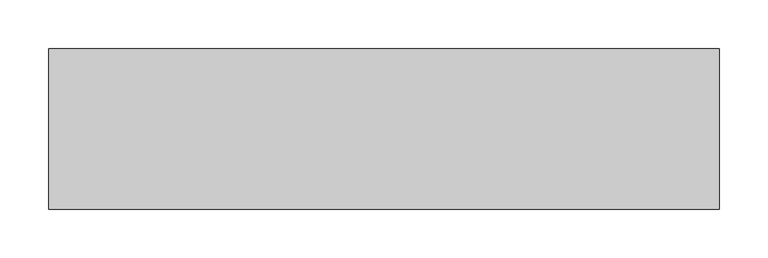
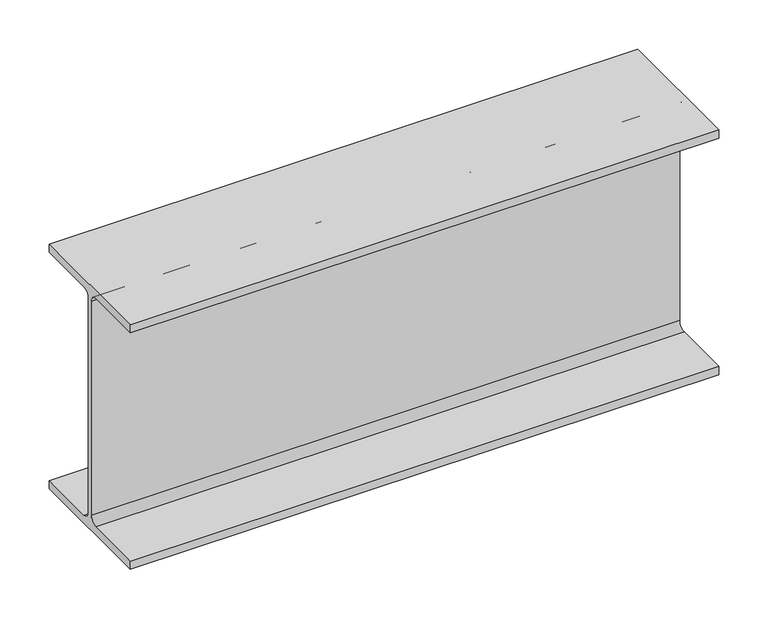
"""IFC4 building model written with IfcOpenShell, lengths in millimetres: beam geometry, Old_Steel Beam_H-KSD3502 : H_SB_ASB_H-300×150x6.5x9."""

import ifcopenshell
import ifcopenshell.guid

model = None  # the IFC model being written
_history = None  # IfcOwnerHistory: only IFC2X3 demands one
_inside = {}  # id of a spatial element -> (the spatial element, [elements in it])
_under = {}  # id of a project, library or spatial element -> (it, [spatial elements below it])
_declared = {}  # id of a project -> (the project, [libraries it declares])
_typed = {}  # id of a type object -> (the type object, [elements of that type])
_made_of = {}  # id of a material, layer set ... -> (it, [elements and type objects made of it])


def new_model(schema):
    """Start an empty IFC model of exactly this schema.

    Asked for "IFC4X3", IfcOpenShell would pick the latest addendum, in which some entities
    have other attributes; the version numbers below select the first issue.
    IFC2X3 requires an IfcOwnerHistory on every rooted entity: one is made here for all.
    """
    global model, _history
    if schema == "IFC4X3":
        model = ifcopenshell.file(schema_version=(4, 3, 0, 0))
    else:
        model = ifcopenshell.file(schema=schema)
    _inside.clear()
    _under.clear()
    _declared.clear()
    _typed.clear()
    _made_of.clear()
    _history = None
    if model.schema == "IFC2X3":
        org = make("IfcOrganization", Name="unknown")
        user = make(
            "IfcPersonAndOrganization",
            ThePerson=make("IfcPerson", FamilyName="unknown"),
            TheOrganization=org,
        )
        app = make(
            "IfcApplication",
            ApplicationDeveloper=org,
            Version="unknown",
            ApplicationFullName="unknown",
            ApplicationIdentifier="unknown",
        )
        _history = make(
            "IfcOwnerHistory",
            OwningUser=user,
            OwningApplication=app,
            ChangeAction="ADDED",
            CreationDate=0,
        )
    return model


def make(cls, **values):
    """One entity of the class cls with the attributes given. An attribute that is None is left unset."""
    return model.create_entity(
        cls, **{name: value for name, value in values.items() if value is not None}
    )


def rooted(cls, **values):
    """An entity with a GlobalId (a new one), such as an element, a storey or a relation."""
    return make(cls, GlobalId=ifcopenshell.guid.new(), OwnerHistory=_history, **values)


def si_unit(unit_type, name, prefix=None):
    """IfcSIUnit, for example si_unit("LENGTHUNIT", "METRE", prefix="MILLI")."""
    return make("IfcSIUnit", UnitType=unit_type, Prefix=prefix, Name=name)


def assignment(units):
    """IfcUnitAssignment: the units of a project."""
    return None if units is None else make("IfcUnitAssignment", Units=units)


def point(xyz):
    """IfcCartesianPoint."""
    return None if xyz is None else make("IfcCartesianPoint", Coordinates=xyz)


def direction(xyz):
    """IfcDirection."""
    return None if xyz is None else make("IfcDirection", DirectionRatios=xyz)


def frame(location, z_axis=None, x_axis=None):
    """IfcAxis2Placement3D, a coordinate frame: its origin and axes. An axis left out is left unset."""
    return make(
        "IfcAxis2Placement3D",
        Location=point(location),
        Axis=direction(z_axis),
        RefDirection=direction(x_axis),
    )


def frame_2d(location, x_axis=None):
    """IfcAxis2Placement2D, a coordinate frame in the plane: its origin and x axis."""
    return make(
        "IfcAxis2Placement2D", Location=point(location), RefDirection=direction(x_axis)
    )


def origin():
    """The frame at (0, 0, 0) with its axes left unset."""
    return frame((0.0, 0.0, 0.0))


def place(relative_to, where):
    """IfcLocalPlacement: puts the frame where relative to a parent placement (None: the world)."""
    return make(
        "IfcLocalPlacement", PlacementRelTo=relative_to, RelativePlacement=where
    )


def context(
    kind, dimensions, precision=None, world=None, true_north=None, identifier=None
):
    """IfcGeometricRepresentationContext, for example the 3D "Model" context."""
    return make(
        "IfcGeometricRepresentationContext",
        ContextIdentifier=identifier,
        ContextType=kind,
        CoordinateSpaceDimension=dimensions,
        Precision=precision,
        WorldCoordinateSystem=world,
        TrueNorth=true_north,
    )


def project(units=None, contexts=None):
    """IfcProject with its units and contexts."""
    return rooted(
        "IfcProject",
        Name="project",
        RepresentationContexts=contexts,
        UnitsInContext=assignment(units),
    )


def spatial(cls, under=None, at=None, **own):
    """A site, building, storey or space (cls), placed at a placement, below another one or the project."""
    s = rooted(cls, ObjectPlacement=at, **own)
    if under is not None:
        _under.setdefault(under.id(), (under, []))[1].append(s)
    return s


def polyline(points):
    """IfcPolyline through the points."""
    return make("IfcPolyline", Points=[point(p) for p in points])


def circle_curve(where, radius):
    """IfcCircle in the frame where."""
    return make("IfcCircle", Position=where, Radius=radius)


def trimmed(basis, trim1, trim2, sense, master):
    """IfcTrimmedCurve: the piece of a basis curve between two trims."""
    return make(
        "IfcTrimmedCurve",
        BasisCurve=basis,
        Trim1=trim1,
        Trim2=trim2,
        SenseAgreement=sense,
        MasterRepresentation=master,
    )


def segment(curve, same_sense, transition):
    """IfcCompositeCurveSegment."""
    return make(
        "IfcCompositeCurveSegment",
        Transition=transition,
        SameSense=same_sense,
        ParentCurve=curve,
    )


def composite_curve(segments, self_intersect=None):
    """IfcCompositeCurve: segments joined end to end."""
    return make("IfcCompositeCurve", Segments=segments, SelfIntersect=self_intersect)


def outline(outer, holes=None, kind="AREA"):
    """IfcArbitraryClosedProfileDef: a profile drawn as a closed curve; with holes, ...WithVoids."""
    if holes is None:
        return make("IfcArbitraryClosedProfileDef", ProfileType=kind, OuterCurve=outer)
    return make(
        "IfcArbitraryProfileDefWithVoids",
        ProfileType=kind,
        OuterCurve=outer,
        InnerCurves=holes,
    )


def extrude(swept, where, along, depth):
    """IfcExtrudedAreaSolid: the profile swept, set in the frame where, extruded along a direction by depth."""
    return make(
        "IfcExtrudedAreaSolid",
        SweptArea=swept,
        Position=where,
        ExtrudedDirection=direction(along),
        Depth=depth,
    )


def shape(context_of_items, identifier, shape_type, items):
    """IfcShapeRepresentation: the items that make up one representation, for example the "Body"."""
    return make(
        "IfcShapeRepresentation",
        ContextOfItems=context_of_items,
        RepresentationIdentifier=identifier,
        RepresentationType=shape_type,
        Items=items,
    )


def source(mapping_origin, context_of_items, identifier, shape_type, items):
    """IfcRepresentationMap: a shape defined once, which mapped items show again and again."""
    return make(
        "IfcRepresentationMap",
        MappingOrigin=mapping_origin,
        MappedRepresentation=shape(context_of_items, identifier, shape_type, items),
    )


def transform(
    local_origin,
    x_axis=None,
    y_axis=None,
    z_axis=None,
    scale=None,
    scale2=None,
    scale3=None,
    uniform=True,
):
    """IfcCartesianTransformationOperator3D, or its non-uniform kind. x_axis, y_axis, z_axis: its Axis1, 2, 3."""
    if uniform:
        return make(
            "IfcCartesianTransformationOperator3D",
            Axis1=direction(x_axis),
            Axis2=direction(y_axis),
            LocalOrigin=point(local_origin),
            Scale=scale,
            Axis3=direction(z_axis),
        )
    return make(
        "IfcCartesianTransformationOperator3DnonUniform",
        Axis1=direction(x_axis),
        Axis2=direction(y_axis),
        LocalOrigin=point(local_origin),
        Scale=scale,
        Axis3=direction(z_axis),
        Scale2=scale2,
        Scale3=scale3,
    )


def mapped(mapping_source, mapping_target):
    """IfcMappedItem: shows the shape of a source again, moved by a transform."""
    return make(
        "IfcMappedItem", MappingSource=mapping_source, MappingTarget=mapping_target
    )


def made_of(thing, what):
    """Note that an element or type object is made of a material, layer set ...; save() writes the relation."""
    if what is not None:
        _made_of.setdefault(what.id(), (what, []))[1].append(thing)
    return thing


def element(
    cls,
    number,
    at=None,
    inside=None,
    cuts=None,
    type_object=None,
    material=None,
    context=None,
    identifier="Body",
    shape_type=None,
    held_by="IfcProductDefinitionShape",
    body=None,
    shapes=None,
    **own,
):
    """One element of the class cls, such as IfcWall. Its Tag is "e" and its number.

    at: its placement. inside: the storey or other place that contains it. cuts: it is an
    opening in that element (IfcRelVoidsElement). A single representation is given by context,
    identifier, shape_type and body (its items); several are given by shapes. held_by: the class
    of the entity that holds the representations. save() writes the other relations.
    """
    e = rooted(cls, Tag="e%d" % number, ObjectPlacement=at, **own)
    if body is not None:
        shapes = [shape(context, identifier, shape_type, body)]
    if shapes is not None:
        e.Representation = make(held_by, Representations=shapes)
    if inside is not None:
        _inside.setdefault(inside.id(), (inside, []))[1].append(e)
    if cuts is not None:
        rooted(
            "IfcRelVoidsElement", RelatingBuildingElement=cuts, RelatedOpeningElement=e
        )
    if type_object is not None:
        _typed.setdefault(type_object.id(), (type_object, []))[1].append(e)
    return made_of(e, material)


def aggregate(whole, parts):
    """IfcRelAggregates: a whole, such as a stair, and the parts it consists of."""
    return rooted("IfcRelAggregates", RelatingObject=whole, RelatedObjects=parts)


def save(model, path):
    """Write the relations noted so far, then the file.

    IfcRelAggregates (storeys below a building ...), IfcRelContainedInSpatialStructure (elements
    in a storey), IfcRelDefinesByType, IfcRelAssociatesMaterial and IfcRelDeclares: one each for
    every whole, place, type object, material and project.
    """
    for whole, parts in _under.values():
        aggregate(whole, parts)
    for where, things in _inside.values():
        rooted(
            "IfcRelContainedInSpatialStructure",
            RelatedElements=things,
            RelatingStructure=where,
        )
    for kind, things in _typed.values():
        rooted("IfcRelDefinesByType", RelatedObjects=things, RelatingType=kind)
    for what, things in _made_of.values():
        rooted("IfcRelAssociatesMaterial", RelatedObjects=things, RelatingMaterial=what)
    for by, libraries in _declared.values():
        rooted("IfcRelDeclares", RelatingContext=by, RelatedDefinitions=libraries)
    model.write(path)


def beam_6268a929(model_context):
    return source(origin(), model_context, "Body", "SweptSolid", [
        extrude(outline(composite_curve([segment(polyline([(82.5, -141.5), (82.5, -151.7), (-82.5, -151.7), (-82.5, -141.5), (-11.9, -141.5)]), True, "CONTINUOUS"), segment(trimmed(circle_curve(frame_2d((-11.9, -132.6)), 8.9), [point((-11.9, -141.5))], [point((-3.0, -132.6))], True, "CARTESIAN"), True, "CONTINUOUS"), segment(polyline([(-3.0, -132.6), (-3.0, 132.6)]), True, "CONTINUOUS"), segment(trimmed(circle_curve(frame_2d((-11.9, 132.6)), 8.9), [point((-3.0, 132.6))], [point((-11.9, 141.5))], True, "CARTESIAN"), True, "CONTINUOUS"), segment(polyline([(-11.9, 141.5), (-82.5, 141.5), (-82.5, 151.7), (82.5, 151.7), (82.5, 141.5), (11.9, 141.5)]), True, "CONTINUOUS"), segment(trimmed(circle_curve(frame_2d((11.9, 132.6)), 8.9), [point((11.9, 141.5))], [point((3.0, 132.6))], True, "CARTESIAN"), True, "CONTINUOUS"), segment(polyline([(3.0, 132.6), (3.0, -132.6)]), True, "CONTINUOUS"), segment(trimmed(circle_curve(frame_2d((11.9, -132.6)), 8.9), [point((3.0, -132.6))], [point((11.9, -141.5))], True, "CARTESIAN"), True, "CONTINUOUS"), segment(polyline([(11.9, -141.5), (82.5, -141.5)]), True, "CONTINUOUS")], self_intersect=False)), frame((-345.0, 0.0, 0.0), z_axis=(1.0, 0.0, 0.0), x_axis=(0.0, 1.0, 0.0)), (0.0, 0.0, 1.0), 689.9999994),
    ])


if __name__ == "__main__":
    model = new_model("IFC4")
    model_context = context("Model", 3, world=origin())
    ifc_project = project(units=[si_unit("LENGTHUNIT", "METRE", prefix="MILLI")], contexts=[model_context])
    site = spatial("IfcSite", under=ifc_project)
    building = spatial("IfcBuilding", under=site)
    placement = place(None, origin())
    beam_shape = beam_6268a929(model_context)
    element("IfcBeam", 1, ObjectType="Old_Steel Beam_H-KSD3502 : H_SB_ASB_H-300×150x6.5x9", at=placement, inside=building, context=model_context, shape_type="MappedRepresentation", body=[
        mapped(beam_shape, transform((0.0, 0.0, 0.0), x_axis=(1.0, 0.0, 0.0), y_axis=(0.0, 1.0, 0.0), z_axis=(0.0, 0.0, 1.0))),
    ])
    save(model, "model.ifc")

# Revit data of these elements
# Type "Old_Steel Beam_H-KSD3502 : H_SB_ASB_H-300×150x6.5x9"
#   Width = 15.0 cm
#   Web Thickness = 0.65 cm
#   Web Fillet = 1.3 cm
#   Warping Constant = 107174.0 cm⁶
#   Torsional Moment of Inertia = 9.9539 cm⁴
#   Torsional Modulus = 1.0 cm³
#   Section Area = 46.78 cm²
#   Plastic Modulus weak axis = 105.0 cm³
#   Plastic Modulus strong axis = 542.0 cm³
#   Perimeter = 1.17 m²/m
#   Nominal Weight = 36.70 kgf/m
#   Moment of Inertia weak axis = 508.00 cm⁴
#   Moment of Inertia strong axis = 7210.00 cm⁴
#   Height = 30.0 cm
#   Flange Thickness = 0.9 cm
#   Elastic Modulus weak axis = 67.7 cm³
#   Elastic Modulus strong axis = 481.0 cm³
#   Centroid Vertical = 15.0 cm
#   Centroid Horizontal = 7.5 cm
#   Length [instance default] = 1.5240 m
#   Structural Material [instance default] = Steel, 45-345
#   Assembly Code = ""
# Element 1 (IfcBeam, "Old_Steel Beam_H-KSD3502 : H_SB_ASB_H-300×150x6.5x9")
#   Structural Material = none
# Materials
#   "Steel, 45-345": class "Metal", colour RGB 189 187 185, transparency 0, Description = "Steel 345 MPa", Cost = 0
